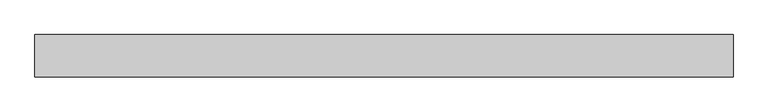
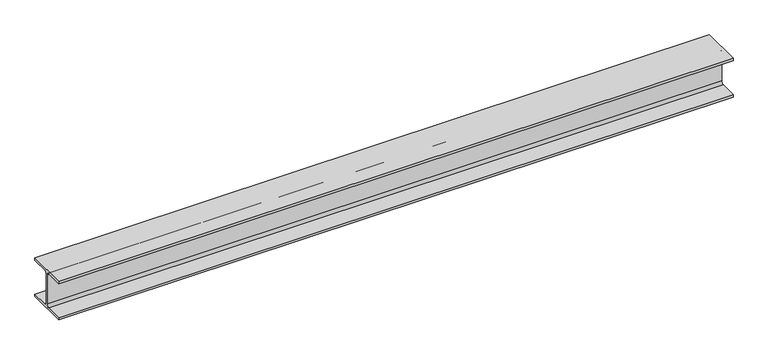
"""IFC4 building model written with IfcOpenShell, lengths in millimetres: beam geometry, 0912_Steel Framing_H-KSD3502 : H_SB_ASB_H-200x200x8x12."""

from ifc_helpers import new_model, si_unit, point, frame, frame_2d, origin, place, context, project, spatial, polyline, circle_curve, trimmed, segment, composite_curve, outline, extrude, source, transform, mapped, element, save


def beam_b610f606(model_context):
    return source(origin(), model_context, "Body", "SweptSolid", [
        extrude(outline(composite_curve([segment(polyline([(100.0, -88.0), (100.0, -100.0), (-100.0, -100.0), (-100.0, -88.0), (-17.0, -88.0)]), True, "CONTINUOUS"), segment(trimmed(circle_curve(frame_2d((-17.0, -75.0)), 13.0), [point((-17.0, -88.0))], [point((-4.0, -75.0))], True, "CARTESIAN"), True, "CONTINUOUS"), segment(polyline([(-4.0, -75.0), (-4.0, 75.0)]), True, "CONTINUOUS"), segment(trimmed(circle_curve(frame_2d((-17.0, 75.0)), 13.0), [point((-4.0, 75.0))], [point((-17.0, 88.0))], True, "CARTESIAN"), True, "CONTINUOUS"), segment(polyline([(-17.0, 88.0), (-100.0, 88.0), (-100.0, 100.0), (100.0, 100.0), (100.0, 88.0), (17.0, 88.0)]), True, "CONTINUOUS"), segment(trimmed(circle_curve(frame_2d((17.0, 75.0)), 13.0), [point((17.0, 88.0))], [point((4.0, 75.0))], True, "CARTESIAN"), True, "CONTINUOUS"), segment(polyline([(4.0, 75.0), (4.0, -75.0)]), True, "CONTINUOUS"), segment(trimmed(circle_curve(frame_2d((17.0, -75.0)), 13.0), [point((4.0, -75.0))], [point((17.0, -88.0))], True, "CARTESIAN"), True, "CONTINUOUS"), segment(polyline([(17.0, -88.0), (100.0, -88.0)]), True, "CONTINUOUS")], self_intersect=False)), frame((-1585.922758, 0.0, 0.0), z_axis=(1.0, 0.0, 0.0), x_axis=(0.0, 1.0, 0.0)), (0.0, 0.0, 1.0), 3299.2628363),
    ])


if __name__ == "__main__":
    model = new_model("IFC4")
    model_context = context("Model", 3, world=origin())
    ifc_project = project(units=[si_unit("LENGTHUNIT", "METRE", prefix="MILLI")], contexts=[model_context])
    site = spatial("IfcSite", under=ifc_project)
    building = spatial("IfcBuilding", under=site)
    placement = place(None, origin())
    beam_shape = beam_b610f606(model_context)
    element("IfcBeam", 1, ObjectType="0912_Steel Framing_H-KSD3502 : H_SB_ASB_H-200x200x8x12", at=placement, inside=building, context=model_context, shape_type="MappedRepresentation", body=[
        mapped(beam_shape, transform((0.0, 0.0, 0.0), x_axis=(1.0, 0.0, 0.0), y_axis=(0.0, 1.0, 0.0), z_axis=(0.0, 0.0, 1.0))),
    ])
    save(model, "model.ifc")

# Revit data of these elements
# Type "0912_Steel Framing_H-KSD3502 : H_SB_ASB_H-200x200x8x12"
#   H_WM Code_1 = "S01AA002-00001 | Main Steel Structure Fabrication Work | Shelter/Building | Medium Steel - Standard (90KG/M>Weight≥30KG/M) | Material: (   )"
#   H_WM Code_2 = "S03AA028-00001 | Main Steel Structure Erection Work | Shelter/Building | Medium Steel (90KG/M>Weight≥30KG/M) | Material: (   )"
#   H_WM Code_3 = "S01AA010-00001 | Main Steel Structure Fabrication Work | Shelter/Building | Steel Painting/Coating | for Non-Fireproofed Steel Surface, Surface Preparation, Primer, Second & Final Coat | Material: (   )"
#   H_Q'ty Cal Type Tag = "SB-Q2"
#   Width = 20.0 cm
#   Web Thickness = 0.8 cm
#   Web Fillet = 1.3 cm
#   Warping Constant = 141000.0 cm⁶
#   W = 0
#   Torsional Moment of Inertia = 26.2485 cm⁴
#   Section Area = 63.53 cm²
#   Plastic Modulus weak axis = 244.0 cm³
#   Plastic Modulus strong axis = 525.0 cm³
#   Perimeter = 1.16 m²/m
#   Nominal Weight = 49.90 kgf/m
#   Moment of Inertia weak axis = 1600.00 cm⁴
#   Moment of Inertia strong axis = 4720.00 cm⁴
#   Height = 20.0 cm
#   Flange Thickness = 1.2 cm
#   Elastic Modulus weak axis = 160.0 cm³
#   Elastic Modulus strong axis = 472.0 cm³
#   Centroid Vertical = 10.0 cm
#   Centroid Horizontal = 10.0 cm
#   Ix = 47200000
#   Length [instance default] = 1.5240 m
#   Zx = 525000
#   b = 0.2000 m
#   h = 0.2000 m
#   r = 0.0130 m
#   s = 0.0080 m
#   t = 0.0120 m
#   A = 0.006353 m²
#   Structural Material [instance default] = Steel, 45-345
#   Assembly Code = ""
# Element 1 (IfcBeam, "0912_Steel Framing_H-KSD3502 : H_SB_ASB_H-200x200x8x12")
#   Structural Material = none
# Materials
#   "Steel, 45-345": class "Metal", colour RGB 189 187 185, transparency 0, Description = "Steel 345 MPa", Cost = 0
